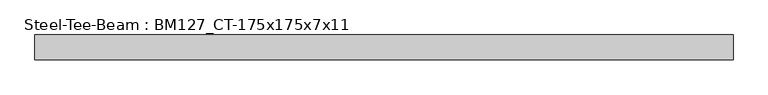
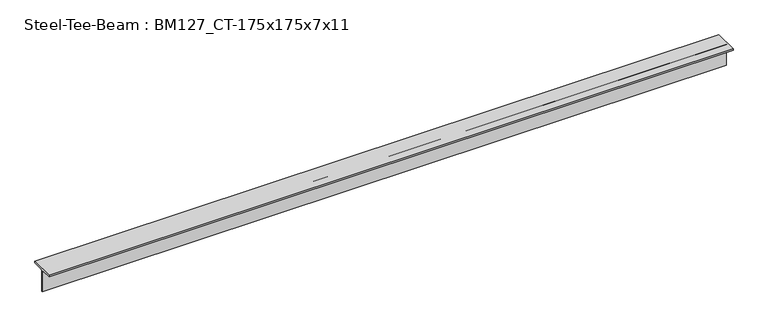
"""IFC4 building model written with IfcOpenShell, lengths in millimetres: beam geometry, Steel-Tee-Beam : BM127_CT-175x175x7x11."""

from ifc_helpers import new_model, si_unit, point, frame, frame_2d, origin, place, context, project, spatial, polyline, circle_curve, trimmed, segment, composite_curve, outline, extrude, source, transform, mapped, element, save


def steel_tee_beam_bm127_ct_175x175x7x11_855b6dfc(model_context):
    return source(origin(), model_context, "Body", "SweptSolid", [
        extrude(outline(composite_curve([segment(polyline([(87.5, 87.5), (87.5, 76.5), (17.5, 76.5)]), True, "CONTINUOUS"), segment(trimmed(circle_curve(frame_2d((17.5, 62.5)), 14.0), [point((17.5, 76.5))], [point((3.5, 62.5))], True, "CARTESIAN"), True, "CONTINUOUS"), segment(polyline([(3.5, 62.5), (3.5, -87.5), (-3.5, -87.5), (-3.5, 62.5)]), True, "CONTINUOUS"), segment(trimmed(circle_curve(frame_2d((-17.5, 62.5)), 14.0), [point((-3.5, 62.5))], [point((-17.5, 76.5))], True, "CARTESIAN"), True, "CONTINUOUS"), segment(polyline([(-17.5, 76.5), (-87.5, 76.5), (-87.5, 87.5), (87.5, 87.5)]), True, "CONTINUOUS")], self_intersect=False)), frame((-2504.4959573, 0.0, 0.0), z_axis=(1.0, 0.0, 0.0), x_axis=(0.0, 1.0, 0.0)), (0.0, 0.0, 1.0), 4880.2539286),
    ])


if __name__ == "__main__":
    model = new_model("IFC4")
    model_context = context("Model", 3, world=origin())
    ifc_project = project(units=[si_unit("LENGTHUNIT", "METRE", prefix="MILLI")], contexts=[model_context])
    site = spatial("IfcSite", under=ifc_project)
    building = spatial("IfcBuilding", under=site)
    placement = place(None, origin())
    steel_tee_beam_bm127_ct_175x175x7x11_shape = steel_tee_beam_bm127_ct_175x175x7x11_855b6dfc(model_context)
    element("IfcBeam", 1, ObjectType="Steel-Tee-Beam : BM127_CT-175x175x7x11", at=placement, inside=building, context=model_context, shape_type="MappedRepresentation", body=[
        mapped(steel_tee_beam_bm127_ct_175x175x7x11_shape, transform((0.0, 0.0, 0.0), x_axis=(1.0, 0.0, 0.0), y_axis=(0.0, 1.0, 0.0), z_axis=(0.0, 0.0, 1.0))),
    ])
    save(model, "model.ifc")

# Revit data of these elements
# Type "Steel-Tee-Beam : BM127_CT-175x175x7x11"
#   Surface Area = 0.00 m²/m
#   Section Area = 31.57 cm²
#   Mass per Unit Length = 24.80 kg/m
#   Length [instance default] = 1524 mm
#   bf = 175 mm
#   d = 175 mm
#   k = 25 mm
#   kr = 14 mm
#   tf = 11 mm
#   tw = 7 mm
#   hec_material4 [instance default] = none
#   hec_material3 [instance default] = none
#   hec_material2 [instance default] = none
#   hec_material1 [instance default] = none
#   Structural Material [instance default] = Steel, 45-345
#   Assembly Code = ""
# Element 1 (IfcBeam, "Steel-Tee-Beam : BM127_CT-175x175x7x11")
#   hec_material3 = F01AC000-00002_Building/Shelter Fire Proofing Work_Intumescent Coating Type_1 hr. rating (UL 1709))
#   hec_material2 = S01AA010-00002_Main Steel Structure Fabrication Work_Shelter/Building_Steel Painting/Coating_for Fireproofed Steel Surface, Surface Preparation & Primer Coat
#   hec_material1 = S03AA029-00001_Main Steel Structure Erection Work_Shelter/Building_Light Steel
#   Structural Material = S01AA003-00001_Main Steel Structure Fabrication Work_Shelter/Building_Light Steel - Standard
#   Materials on its faces: "S01AA003-00001_Main Steel Structure Fabrication Work_Shelter/Building_Light Steel - Standard"
# Materials
#   "Steel, 45-345": class "Metal", colour RGB 189 187 185, transparency 0, Description = "Steel 345 MPa", Cost = 0
#   "S01AA003-00001_Main Steel Structure Fabrication Work_Shelter/Building_Light Steel - Standard": class "Metal", colour RGB 120 120 120, transparency 0, Comments = "(30KG/M>Weight)", Description = "Structural steel 50ksi", W00) Work Master Code = "S01AA003-00001", W01) Work Master_Lv1 = "Main Steel Structure Fabrication Work", W02) Work Master_Lv2 = "Shelter/Building", W03) Work Master_Spec.1 = "Light Steel - Standard (30KG/M>Weight)", Cost = 0
#   "F01AC000-00002_Building/Shelter Fire Proofing Work_Intumescent Coating Type_1 hr. rating (UL 1709))": class "Metal", colour RGB 255 128 128, transparency 0, Description = "Paint finished steel", W00) Work Master Code = "F01AC000-00002", W01) Work Master_Lv1 = "Building/Shelter Fire Proofing Work", W02) Work Master_Lv2 = "Intumescent Coating Type", W03) Work Master_Spec.1 = "1 hr. rating (UL 1709)", Cost = 0
#   "S01AA010-00002_Main Steel Structure Fabrication Work_Shelter/Building_Steel Painting/Coating_for Fireproofed Steel Surface, Surface Preparation & Primer Coat": class "Metal", colour RGB 120 120 120, transparency 0, Description = "Paint finished steel", W00) Work Master Code = "SS01AA010-00002", W01) Work Master_Lv1 = "Main Steel Structure Fabrication Work", W02) Work Master_Lv2 = "Shelter/Building", W03) Work Master_Spec.1 = "Steel Painting/Coating", W04) Work Master_Spec.2 = "for Fireproofed Steel Surface, Surface Preparation & Primer Coat", Cost = 0
#   "S03AA029-00001_Main Steel Structure Erection Work_Shelter/Building_Light Steel": class "Metal", colour RGB 120 120 120, transparency 0, Comments = "(30KG/M>Weight)", Description = "Structural steel 50ksi", W00) Work Master Code = "S03AA029-00001", W01) Work Master_Lv1 = "Main Steel Structure Erection Work", W02) Work Master_Lv2 = "Shelter/Building", W03) Work Master_Spec.1 = "Light Steel (30KG/M>Weight)", Cost = 0
